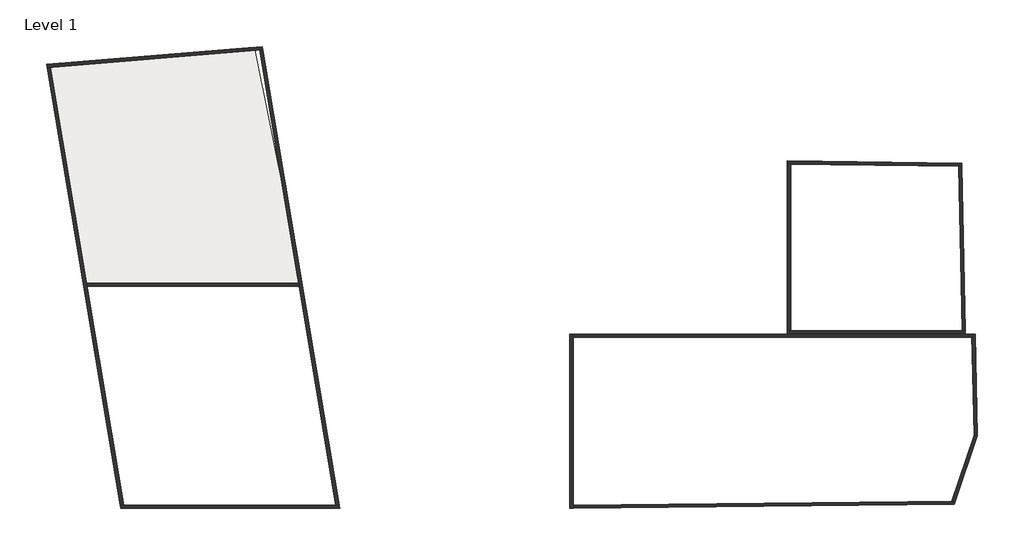
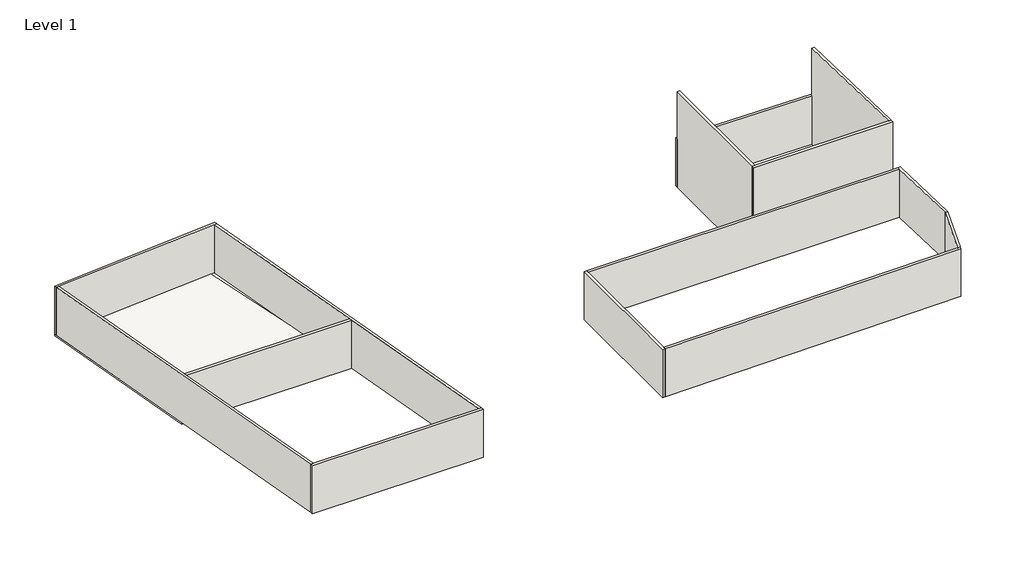
# One storey: 14 walls, 1 slab.
"""IFC4 building model written with IfcOpenShell, lengths in millimetres."""

from ifc_helpers import new_model, si_unit, frame, origin, origin_with_axes, place, context, project, spatial, polyline, outline, extrude, faceted_brep, element, save

model = new_model("IFC4")

# Units and contexts
model_context = context("Model", 3, world=origin())
ifc_project = project(units=[si_unit("LENGTHUNIT", "METRE", prefix="MILLI")], contexts=[model_context])

# Site, building, storey
site = spatial("IfcSite", under=ifc_project)
building = spatial("IfcBuilding", under=site)
storey = spatial("IfcBuildingStorey", under=building, Name="Level 1", Elevation=0.0)

# Slab
placement = place(None, origin())
element("IfcSlab", 1, ObjectType="Generic 150mm", at=placement, inside=storey, context=model_context, shape_type="SweptSolid", body=[
    extrude(outline(polyline([(-13925.0882564, 14998.0535577), (-10978.6328891, 464.9901881), (-24463.1749, 464.9901881), (-26716.4215745, 13944.3927249), (-13925.0882564, 14998.0535577)])), frame((0.0, 0.0, -150.0), z_axis=(0.0, 0.0, 1.0), x_axis=(1.0, 0.0, 0.0)), (0.0, 0.0, 1.0), 150.0),
])

# Walls
element("IfcWall", 2, ObjectType="Generic - 200mm", at=placement, inside=storey, context=model_context, shape_type="Brep", body=[
    faceted_brep([(-26683.3315384, 13746.4410669, 0.0), (-26483.310689, 13762.9173895, 0.0), (-13581.965904, 14825.6401998, 0.0), (-13381.9450546, 14842.1165224, 0.0), (-13381.9450546, 14842.1165224, 4000.0), (-13581.965904, 14825.6401998, 4000.0), (-26483.310689, 13762.9173895, 4000.0), (-26683.3315384, 13746.4410669, 4000.0), (-26716.4215744, 13944.3927249, 0.0), (-26716.4215744, 13944.3927249, 4000.0), (-13415.0350906, 15040.0681804, 4000.0), (-13415.0350906, 15040.0681804, 0.0)], [[[0, 1, 2, 3, 4, 5, 6, 7]], [[8, 9, 10, 11]], [[3, 2, 1, 0, 8, 11]], [[7, 6, 5, 4, 10, 9]], [[4, 3, 11, 10]], [[0, 7, 9, 8]]]),
])
element("IfcWall", 3, ObjectType="Generic - 200mm", at=placement, inside=storey, context=model_context, shape_type="Brep", body=[
    faceted_brep([(-13581.965904, 14825.6401998, 0.0), (-11181.4079569, 464.9901881, 0.0), (-11147.9755155, 264.9901881, 0.0), (-8894.6289678, -13215.0098119, 0.0), (-8894.6289678, -13215.0098119, 4000.0), (-11147.9755155, 264.9901881, 4000.0), (-11181.4079569, 464.9901881, 4000.0), (-13581.965904, 14825.6401998, 4000.0), (-13381.9450546, 14842.1165224, 0.0), (-13381.9450546, 14842.1165224, 4000.0), (-8691.8539, -13215.0098119, 4000.0), (-8691.8539, -13215.0098119, 0.0)], [[[0, 1, 2, 3, 4, 5, 6, 7]], [[8, 9, 10, 11]], [[3, 2, 1, 0, 8, 11]], [[7, 6, 5, 4, 10, 9]], [[0, 7, 9, 8]], [[4, 3, 11, 10]]]),
])
element("IfcWall", 4, ObjectType="Generic - 200mm", at=placement, inside=storey, context=model_context, shape_type="SweptSolid", body=[
    extrude(outline(polyline([(-24260.3998321, 464.9901881), (-11181.4079569, 464.9901881), (-11147.9755155, 264.9901881), (-24226.9673908, 264.9901881), (-24260.3998321, 464.9901881)])), origin_with_axes(), (0.0, 0.0, 1.0), 4000.0),
])
element("IfcWall", 5, ObjectType="Generic - 200mm", at=placement, inside=storey, context=model_context, shape_type="Brep", body=[
    faceted_brep([(-21973.6208431, -13215.0098119, 0.0), (-24226.9673908, 264.9901881, 0.0), (-24260.3998321, 464.9901881, 0.0), (-26483.310689, 13762.9173895, 0.0), (-26483.310689, 13762.9173895, 4000.0), (-24260.3998321, 464.9901881, 4000.0), (-24226.9673908, 264.9901881, 4000.0), (-21973.6208431, -13215.0098119, 4000.0), (-22176.395911, -13215.0098119, 0.0), (-22176.395911, -13215.0098119, 4000.0), (-26683.3315384, 13746.4410669, 4000.0), (-26683.3315384, 13746.4410669, 0.0)], [[[0, 1, 2, 3, 4, 5, 6, 7]], [[8, 9, 10, 11]], [[3, 2, 1, 0, 8, 11]], [[7, 6, 5, 4, 10, 9]], [[4, 3, 11, 10]], [[0, 7, 9, 8]]]),
])
element("IfcWall", 6, ObjectType="Generic - 200mm", at=placement, inside=storey, context=model_context, shape_type="Brep", body=[
    faceted_brep([(-22142.9634696, -13415.0098119, 0.0), (-8658.4214586, -13415.0098119, 0.0), (-8658.4214586, -13415.0098119, 4000.0), (-22142.9634696, -13415.0098119, 4000.0), (-22176.395911, -13215.0098119, 0.0), (-22176.395911, -13215.0098119, 4000.0), (-21973.6208431, -13215.0098119, 4000.0), (-8894.6289678, -13215.0098119, 4000.0), (-8691.8539, -13215.0098119, 4000.0), (-8691.8539, -13215.0098119, 0.0), (-8894.6289678, -13215.0098119, 0.0), (-21973.6208431, -13215.0098119, 0.0)], [[[0, 1, 2, 3]], [[4, 5, 6, 7, 8, 9, 10, 11]], [[1, 0, 4, 11, 10, 9]], [[3, 2, 8, 7, 6, 5]], [[2, 1, 9, 8]], [[0, 3, 5, 4]]]),
])
element("IfcWall", 7, ObjectType="Generic - 200mm", at=placement, inside=storey, context=model_context, shape_type="Brep", body=[
    faceted_brep([(30634.9948132, -8930.080328, 0.0), (30497.5685349, -2673.3672809, 0.0), (30497.5685349, -2673.3672809, 4000.0), (30634.9948132, -8930.080328, 4000.0), (30434.2733115, -8899.4281518, 0.0), (30434.2733115, -8899.4281518, 4000.0), (30301.9132189, -2873.3672809, 4000.0), (30297.5202963, -2673.3672809, 4000.0), (30297.5202963, -2673.3672809, 0.0), (30301.9132189, -2873.3672809, 0.0)], [[[0, 1, 2, 3]], [[4, 5, 6, 7, 8, 9]], [[1, 0, 4, 9, 8]], [[3, 2, 7, 6, 5]], [[0, 3, 5, 4]], [[2, 1, 8, 7]]]),
])
element("IfcWall", 8, ObjectType="Generic - 200mm", at=placement, inside=storey, context=model_context, shape_type="Brep", body=[
    faceted_brep([(29666.179537, 7854.6709857, 0.0), (18923.716007, 7998.5119409, 0.0), (18923.716007, 7998.5119409, 4000.0), (29666.179537, 7854.6709857, 4000.0), (29670.5741458, 7654.5942139, 0.0), (29670.5741458, 7654.5942139, 4000.0), (18923.716007, 7798.4940126, 4000.0), (18923.716007, 7798.4940126, 0.0), (19123.716007, 7795.8160244, 0.0), (29470.4670547, 7657.273636, 0.0)], [[[0, 1, 2, 3]], [[4, 5, 6, 7, 8, 9]], [[1, 0, 4, 9, 8, 7]], [[3, 2, 6, 5]], [[2, 1, 7, 6]], [[0, 3, 5, 4]]]),
])
element("IfcWall", 9, ObjectType="Generic - 200mm", at=placement, inside=storey, context=model_context, shape_type="Brep", body=[
    faceted_brep([(5523.716007, -2673.3672809, 0.0), (5523.716007, -13410.9526121, 0.0), (5523.716007, -13410.9526121, 4000.0), (5523.716007, -2673.3672809, 4000.0), (5723.716007, -2673.3672809, 0.0), (5723.716007, -2673.3672809, 4000.0), (5723.716007, -2873.3672809, 4000.0), (5723.716007, -13208.9137243, 4000.0), (5723.716007, -13408.9240121, 4000.0), (5723.716007, -13408.9240121, 0.0), (5723.716007, -13208.9137243, 0.0), (5723.716007, -2873.3672809, 0.0)], [[[0, 1, 2, 3]], [[4, 5, 6, 7, 8, 9, 10, 11]], [[1, 0, 4, 11, 10, 9]], [[3, 2, 8, 7, 6, 5]], [[2, 1, 9, 8]], [[0, 3, 5, 4]]]),
])
element("IfcWall", 10, ObjectType="Generic - 200mm", at=placement, inside=storey, context=model_context, shape_type="Brep", body=[
    faceted_brep([(5723.716007, -13408.9240121, 0.0), (29205.9259587, -13170.7439642, 0.0), (29205.9259587, -13170.7439642, 4000.0), (5723.716007, -13408.9240121, 4000.0), (5723.716007, -13208.9137243, 0.0), (5723.716007, -13208.9137243, 4000.0), (29061.7840586, -12972.1957077, 4000.0), (29273.5589617, -12970.0476749, 4000.0), (29273.5589617, -12970.0476749, 0.0), (29061.7840586, -12972.1957077, 0.0)], [[[0, 1, 2, 3]], [[4, 5, 6, 7, 8, 9]], [[1, 0, 4, 9, 8]], [[3, 2, 7, 6, 5]], [[0, 3, 5, 4]], [[2, 1, 8, 7]]]),
])
element("IfcWall", 11, ObjectType="Generic - 200mm", at=placement, inside=storey, context=model_context, shape_type="SweptSolid", body=[
    extrude(outline(polyline([(30634.9948132, -8930.080328), (29273.5589617, -12970.0476749), (29061.7840586, -12972.1957077), (30434.2733115, -8899.4281518), (30634.9948132, -8930.080328)])), origin_with_axes(), (0.0, 0.0, 1.0), 4000.0),
])
element("IfcWall", 12, ObjectType="Generic - 200mm", at=placement, inside=storey, context=model_context, shape_type="SweptSolid", body=[
    extrude(outline(polyline([(30301.9132189, -2873.3672809), (5723.716007, -2873.3672809), (5723.716007, -2673.3672809), (30297.5202963, -2673.3672809), (30301.9132189, -2873.3672809)])), origin_with_axes(), (0.0, 0.0, 1.0), 4000.0),
])
element("IfcWall", 13, ObjectType="Generic - 200mm", at=placement, inside=storey, context=model_context, shape_type="Brep", body=[
    faceted_brep([(29893.0308966, -2473.3672809, 0.0), (29692.982658, -2473.3672809, 0.0), (19123.716007, -2473.3672809, 0.0), (18923.716007, -2473.3672809, 0.0), (18923.716007, -2473.3672809, 8000.0), (19123.716007, -2473.3672809, 8000.0), (29692.982658, -2473.3672809, 8000.0), (29893.0308966, -2473.3672809, 8000.0), (29897.4238191, -2673.3672809, 0.0), (29897.4238191, -2673.3672809, 8000.0), (18923.716007, -2673.3672809, 8000.0), (18923.716007, -2673.3672809, 0.0)], [[[0, 1, 2, 3, 4, 5, 6, 7]], [[8, 9, 10, 11]], [[3, 2, 1, 0, 8, 11]], [[7, 6, 5, 4, 10, 9]], [[4, 3, 11, 10]], [[0, 7, 9, 8]]]),
])
element("IfcWall", 14, ObjectType="Generic - 200mm", at=placement, inside=storey, context=model_context, shape_type="Brep", body=[
    faceted_brep([(19123.716007, -2473.3672809, 0.0), (19123.716007, 7795.8160244, 0.0), (19123.716007, 7795.8160244, 8000.0), (19123.716007, -2473.3672809, 8000.0), (18923.716007, -2473.3672809, 0.0), (18923.716007, -2473.3672809, 8000.0), (18923.716007, 7798.4940126, 8000.0), (18923.716007, 7798.4940126, 4000.0), (18923.716007, 7798.4940126, 0.0)], [[[0, 1, 2, 3]], [[4, 5, 6, 7, 8]], [[1, 0, 4, 8]], [[3, 2, 6, 5]], [[2, 1, 8, 7, 6]], [[0, 3, 5, 4]]]),
])
element("IfcWall", 15, ObjectType="Generic - 200mm", at=placement, inside=storey, context=model_context, shape_type="Brep", body=[
    faceted_brep([(29893.0308966, -2473.3672809, 0.0), (29670.5741458, 7654.5942139, 0.0), (29670.5741458, 7654.5942139, 4000.0), (29670.5741458, 7654.5942139, 8000.0), (29893.0308966, -2473.3672809, 8000.0), (29692.982658, -2473.3672809, 0.0), (29692.982658, -2473.3672809, 8000.0), (29470.4670547, 7657.273636, 8000.0), (29470.4670547, 7657.273636, 0.0)], [[[0, 1, 2, 3, 4]], [[5, 6, 7, 8]], [[1, 0, 5, 8]], [[4, 3, 7, 6]], [[3, 2, 1, 8, 7]], [[0, 4, 6, 5]]]),
])

save(model, "model.ifc")

# Revit data of these elements
# Project information
#   Project Issue Date = "Issue Date"
#   Project Status = "Project Status"
#   Client Name = "Owner"
#   Project Address = "Enter address here"
#   Project Name = "Project Name"
#   Project Number = "0001"
# Type "Generic 150mm"
#   Function = 0
#   Layers, outside or top first: 15 cm no material (function 1)
# Type "Generic - 200mm"
#   Layers, outside or top first: 20 cm no material (function 1)
# Element 1 (IfcSlab, "Generic 150mm")
#   built-in parameter 1001955 = 0.0821875 (stored number, unit not read)
#   Height Offset From Level = 0 cm
#   Phase Created = New Construction
#   Materials on its faces: "Default Floor"
# Elements 2, 3, 4, 5, 6, 7, 8, 9, 10, 11, 12 (IfcWall, "Generic - 200mm")
#   Top Offset = 0 cm
#   Base Offset = 0 cm
#   wall height = 400 cm
#   Phase Created = New Construction
#   Base Constraint = Level 1
#   Top Constraint = Level 2
#   Materials on its faces: "Default Wall"
# Elements 13, 14, 15 (IfcWall, "Generic - 200mm")
#   Top Offset = 0 cm
#   Base Offset = 0 cm
#   Unconnected Height = 800 cm
#   wall height = 800 cm
#   Phase Created = New Construction
#   Base Constraint = Level 1
#   Materials on its faces: "Default Wall"
# Materials
#   "Default Floor": class "Miscellaneous", colour RGB 127 127 127, transparency 0, Cost = 0
#   "Default Wall": class "Miscellaneous", colour RGB 128 128 128, transparency 0, Cost = 0
# Room at (21170.766, 2310.514) mm, phase "New Construction", upper level "Level 1", upper offset 243.84 cm, lower offset 0 cm
#   Number = "5"
#   Name = "Room"
# Room at (-16901.249, -6463.461) mm, phase "New Construction", upper level "Level 1", upper offset 243.84 cm, lower offset 0 cm
#   Number = "6"
#   Name = "Room"
# Area at (18053.034, -7004.344) mm, upper offset 243.84 cm, lower offset 0 cm
#   Number = "2"
#   Name = "Area"
# Room, not placed, phase "New Construction", upper offset 0 cm, lower offset 0 cm
#   Number = "1"
#   Name = "Room"
# Room at (-5775.751, 4520.425) mm, phase "New Construction", upper level "Level 1", upper offset 400 cm, lower offset 0 cm
#   Number = "2"
#   Name = "Room"
# Room at (11926.664, -3323.192) mm, phase "New Construction", upper level "Level 1", upper offset 400 cm, lower offset 0 cm
#   Number = "3"
#   Name = "Room"
# Room, not placed, phase "New Construction", upper offset 0 cm, lower offset 0 cm
#   Number = "4"
#   Name = "Room"
# Area, not placed, upper offset 0 cm, lower offset 0 cm
#   Number = "1"
#   Name = "Area"
